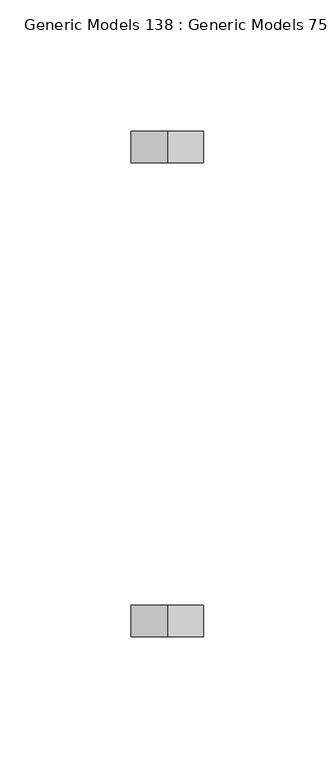
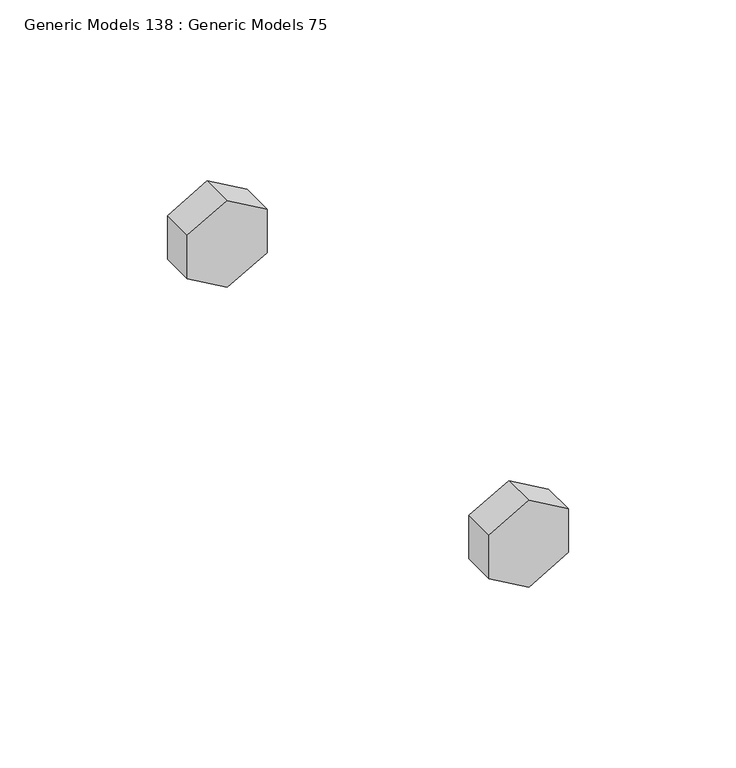
"""IFC4 building model written with IfcOpenShell, lengths in millimetres: proxy geometry, Generic Models 138 : Generic Models 75."""

import ifcopenshell
import ifcopenshell.guid

model = None  # the IFC model being written
_history = None  # IfcOwnerHistory: only IFC2X3 demands one
_inside = {}  # id of a spatial element -> (the spatial element, [elements in it])
_under = {}  # id of a project, library or spatial element -> (it, [spatial elements below it])
_declared = {}  # id of a project -> (the project, [libraries it declares])
_typed = {}  # id of a type object -> (the type object, [elements of that type])
_made_of = {}  # id of a material, layer set ... -> (it, [elements and type objects made of it])


def new_model(schema):
    """Start an empty IFC model of exactly this schema.

    Asked for "IFC4X3", IfcOpenShell would pick the latest addendum, in which some entities
    have other attributes; the version numbers below select the first issue.
    IFC2X3 requires an IfcOwnerHistory on every rooted entity: one is made here for all.
    """
    global model, _history
    if schema == "IFC4X3":
        model = ifcopenshell.file(schema_version=(4, 3, 0, 0))
    else:
        model = ifcopenshell.file(schema=schema)
    _inside.clear()
    _under.clear()
    _declared.clear()
    _typed.clear()
    _made_of.clear()
    _history = None
    if model.schema == "IFC2X3":
        org = make("IfcOrganization", Name="unknown")
        user = make(
            "IfcPersonAndOrganization",
            ThePerson=make("IfcPerson", FamilyName="unknown"),
            TheOrganization=org,
        )
        app = make(
            "IfcApplication",
            ApplicationDeveloper=org,
            Version="unknown",
            ApplicationFullName="unknown",
            ApplicationIdentifier="unknown",
        )
        _history = make(
            "IfcOwnerHistory",
            OwningUser=user,
            OwningApplication=app,
            ChangeAction="ADDED",
            CreationDate=0,
        )
    return model


def make(cls, **values):
    """One entity of the class cls with the attributes given. An attribute that is None is left unset."""
    return model.create_entity(
        cls, **{name: value for name, value in values.items() if value is not None}
    )


def rooted(cls, **values):
    """An entity with a GlobalId (a new one), such as an element, a storey or a relation."""
    return make(cls, GlobalId=ifcopenshell.guid.new(), OwnerHistory=_history, **values)


def si_unit(unit_type, name, prefix=None):
    """IfcSIUnit, for example si_unit("LENGTHUNIT", "METRE", prefix="MILLI")."""
    return make("IfcSIUnit", UnitType=unit_type, Prefix=prefix, Name=name)


def assignment(units):
    """IfcUnitAssignment: the units of a project."""
    return None if units is None else make("IfcUnitAssignment", Units=units)


def point(xyz):
    """IfcCartesianPoint."""
    return None if xyz is None else make("IfcCartesianPoint", Coordinates=xyz)


def direction(xyz):
    """IfcDirection."""
    return None if xyz is None else make("IfcDirection", DirectionRatios=xyz)


def frame(location, z_axis=None, x_axis=None):
    """IfcAxis2Placement3D, a coordinate frame: its origin and axes. An axis left out is left unset."""
    return make(
        "IfcAxis2Placement3D",
        Location=point(location),
        Axis=direction(z_axis),
        RefDirection=direction(x_axis),
    )


def origin():
    """The frame at (0, 0, 0) with its axes left unset."""
    return frame((0.0, 0.0, 0.0))


def place(relative_to, where):
    """IfcLocalPlacement: puts the frame where relative to a parent placement (None: the world)."""
    return make(
        "IfcLocalPlacement", PlacementRelTo=relative_to, RelativePlacement=where
    )


def context(
    kind, dimensions, precision=None, world=None, true_north=None, identifier=None
):
    """IfcGeometricRepresentationContext, for example the 3D "Model" context."""
    return make(
        "IfcGeometricRepresentationContext",
        ContextIdentifier=identifier,
        ContextType=kind,
        CoordinateSpaceDimension=dimensions,
        Precision=precision,
        WorldCoordinateSystem=world,
        TrueNorth=true_north,
    )


def project(units=None, contexts=None):
    """IfcProject with its units and contexts."""
    return rooted(
        "IfcProject",
        Name="project",
        RepresentationContexts=contexts,
        UnitsInContext=assignment(units),
    )


def spatial(cls, under=None, at=None, **own):
    """A site, building, storey or space (cls), placed at a placement, below another one or the project."""
    s = rooted(cls, ObjectPlacement=at, **own)
    if under is not None:
        _under.setdefault(under.id(), (under, []))[1].append(s)
    return s


def polyline(points):
    """IfcPolyline through the points."""
    return make("IfcPolyline", Points=[point(p) for p in points])


def outline(outer, holes=None, kind="AREA"):
    """IfcArbitraryClosedProfileDef: a profile drawn as a closed curve; with holes, ...WithVoids."""
    if holes is None:
        return make("IfcArbitraryClosedProfileDef", ProfileType=kind, OuterCurve=outer)
    return make(
        "IfcArbitraryProfileDefWithVoids",
        ProfileType=kind,
        OuterCurve=outer,
        InnerCurves=holes,
    )


def extrude(swept, where, along, depth):
    """IfcExtrudedAreaSolid: the profile swept, set in the frame where, extruded along a direction by depth."""
    return make(
        "IfcExtrudedAreaSolid",
        SweptArea=swept,
        Position=where,
        ExtrudedDirection=direction(along),
        Depth=depth,
    )


def shape(context_of_items, identifier, shape_type, items):
    """IfcShapeRepresentation: the items that make up one representation, for example the "Body"."""
    return make(
        "IfcShapeRepresentation",
        ContextOfItems=context_of_items,
        RepresentationIdentifier=identifier,
        RepresentationType=shape_type,
        Items=items,
    )


def source(mapping_origin, context_of_items, identifier, shape_type, items):
    """IfcRepresentationMap: a shape defined once, which mapped items show again and again."""
    return make(
        "IfcRepresentationMap",
        MappingOrigin=mapping_origin,
        MappedRepresentation=shape(context_of_items, identifier, shape_type, items),
    )


def transform(
    local_origin,
    x_axis=None,
    y_axis=None,
    z_axis=None,
    scale=None,
    scale2=None,
    scale3=None,
    uniform=True,
):
    """IfcCartesianTransformationOperator3D, or its non-uniform kind. x_axis, y_axis, z_axis: its Axis1, 2, 3."""
    if uniform:
        return make(
            "IfcCartesianTransformationOperator3D",
            Axis1=direction(x_axis),
            Axis2=direction(y_axis),
            LocalOrigin=point(local_origin),
            Scale=scale,
            Axis3=direction(z_axis),
        )
    return make(
        "IfcCartesianTransformationOperator3DnonUniform",
        Axis1=direction(x_axis),
        Axis2=direction(y_axis),
        LocalOrigin=point(local_origin),
        Scale=scale,
        Axis3=direction(z_axis),
        Scale2=scale2,
        Scale3=scale3,
    )


def mapped(mapping_source, mapping_target):
    """IfcMappedItem: shows the shape of a source again, moved by a transform."""
    return make(
        "IfcMappedItem", MappingSource=mapping_source, MappingTarget=mapping_target
    )


def made_of(thing, what):
    """Note that an element or type object is made of a material, layer set ...; save() writes the relation."""
    if what is not None:
        _made_of.setdefault(what.id(), (what, []))[1].append(thing)
    return thing


def element(
    cls,
    number,
    at=None,
    inside=None,
    cuts=None,
    type_object=None,
    material=None,
    context=None,
    identifier="Body",
    shape_type=None,
    held_by="IfcProductDefinitionShape",
    body=None,
    shapes=None,
    **own,
):
    """One element of the class cls, such as IfcWall. Its Tag is "e" and its number.

    at: its placement. inside: the storey or other place that contains it. cuts: it is an
    opening in that element (IfcRelVoidsElement). A single representation is given by context,
    identifier, shape_type and body (its items); several are given by shapes. held_by: the class
    of the entity that holds the representations. save() writes the other relations.
    """
    e = rooted(cls, Tag="e%d" % number, ObjectPlacement=at, **own)
    if body is not None:
        shapes = [shape(context, identifier, shape_type, body)]
    if shapes is not None:
        e.Representation = make(held_by, Representations=shapes)
    if inside is not None:
        _inside.setdefault(inside.id(), (inside, []))[1].append(e)
    if cuts is not None:
        rooted(
            "IfcRelVoidsElement", RelatingBuildingElement=cuts, RelatedOpeningElement=e
        )
    if type_object is not None:
        _typed.setdefault(type_object.id(), (type_object, []))[1].append(e)
    return made_of(e, material)


def aggregate(whole, parts):
    """IfcRelAggregates: a whole, such as a stair, and the parts it consists of."""
    return rooted("IfcRelAggregates", RelatingObject=whole, RelatedObjects=parts)


def save(model, path):
    """Write the relations noted so far, then the file.

    IfcRelAggregates (storeys below a building ...), IfcRelContainedInSpatialStructure (elements
    in a storey), IfcRelDefinesByType, IfcRelAssociatesMaterial and IfcRelDeclares: one each for
    every whole, place, type object, material and project.
    """
    for whole, parts in _under.values():
        aggregate(whole, parts)
    for where, things in _inside.values():
        rooted(
            "IfcRelContainedInSpatialStructure",
            RelatedElements=things,
            RelatingStructure=where,
        )
    for kind, things in _typed.values():
        rooted("IfcRelDefinesByType", RelatedObjects=things, RelatingType=kind)
    for what, things in _made_of.values():
        rooted("IfcRelAssociatesMaterial", RelatedObjects=things, RelatingMaterial=what)
    for by, libraries in _declared.values():
        rooted("IfcRelDeclares", RelatingContext=by, RelatedDefinitions=libraries)
    model.write(path)


def generic_models_138_generic_models_75_b34d7099(model_context):
    return source(origin(), model_context, "Body", "SweptSolid", [
        extrude(outline(polyline([(268689.2902933, 31974.4067029), (268673.4537198, 31974.4067029), (268665.535433, 31988.1215778), (268673.4537198, 32001.8364528), (268689.2902933, 32001.8364528), (268697.20858, 31988.1215778), (268689.2902933, 31974.4067029)])), frame((0.0, 36491.5582942, 0.0), z_axis=(0.0, 1.0, 0.0), x_axis=(0.0, 0.0, 1.0)), (0.0, 0.0, 1.0), 11.90625),
        extrude(outline(polyline([(268689.2902933, 31974.4067029), (268673.4537198, 31974.4067029), (268665.535433, 31988.1215778), (268673.4537198, 32001.8364528), (268689.2902933, 32001.8364528), (268697.20858, 31988.1215778), (268689.2902933, 31974.4067029)])), frame((0.0, 36311.3770442, 0.0), z_axis=(0.0, 1.0, 0.0), x_axis=(0.0, 0.0, 1.0)), (0.0, 0.0, 1.0), 11.90625),
    ])


if __name__ == "__main__":
    model = new_model("IFC4")
    model_context = context("Model", 3, world=origin())
    ifc_project = project(units=[si_unit("LENGTHUNIT", "METRE", prefix="MILLI")], contexts=[model_context])
    site = spatial("IfcSite", under=ifc_project)
    building = spatial("IfcBuilding", under=site)
    placement = place(None, origin())
    generic_models_138_generic_models_75_shape = generic_models_138_generic_models_75_b34d7099(model_context)
    element("IfcBuildingElementProxy", 1, Name="Generic Models 138 : Generic Models 75", ObjectType="Generic Models 138 : Generic Models 75", at=placement, inside=building, context=model_context, shape_type="MappedRepresentation", body=[
        mapped(generic_models_138_generic_models_75_shape, transform((0.0, 0.0, 0.0), x_axis=(1.0, 0.0, 0.0), y_axis=(0.0, 1.0, 0.0), z_axis=(0.0, 0.0, 1.0))),
    ])
    save(model, "model.ifc")

# Revit data of these elements
# Element 1 (IfcBuildingElementProxy, "Generic Models 138 : Generic Models 75")
#   Materials on its faces: "3/4\" GALV. THRU BOLTS"
# Materials
#   "3/4\" GALV. THRU BOLTS": class "Generic", colour RGB 105 69 171, transparency 0, Cost = 0
